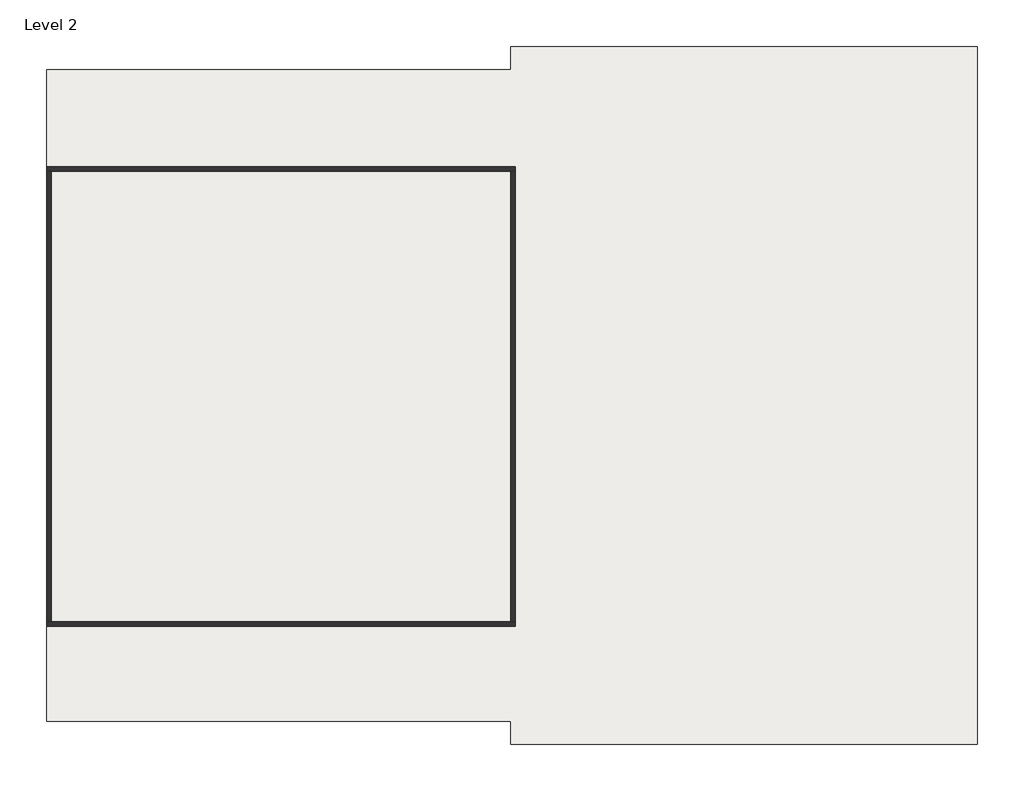
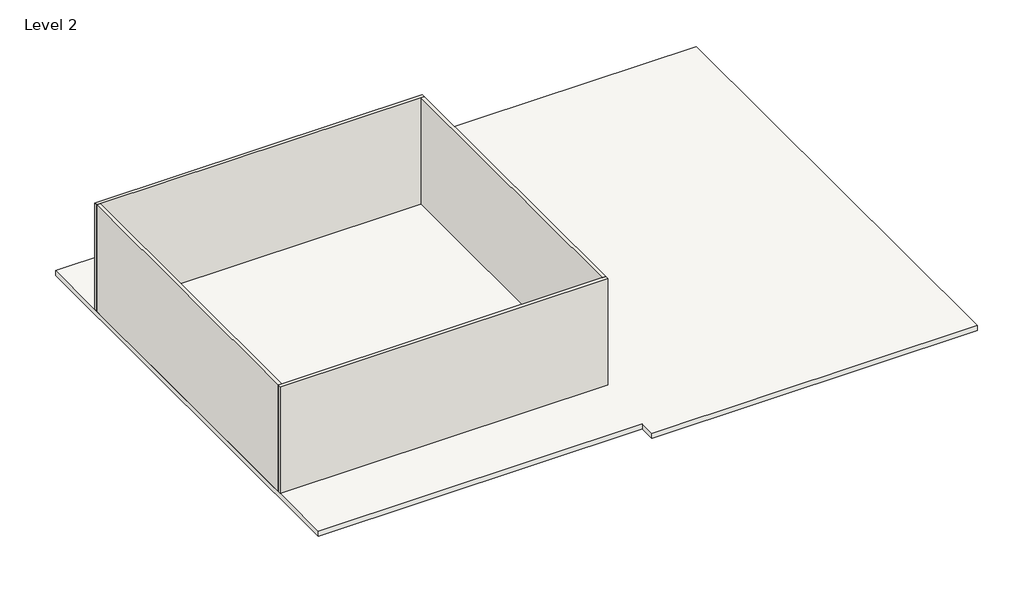
# One storey: 4 walls, 1 slab.
"""IFC4 building model written with IfcOpenShell, lengths in millimetres."""

from ifc_helpers import new_model, si_unit, frame, origin, place, context, project, spatial, polyline, outline, extrude, faceted_brep, element, save

model = new_model("IFC4")

# Units and contexts
model_context = context("Model", 3, world=origin())
ifc_project = project(units=[si_unit("LENGTHUNIT", "METRE", prefix="MILLI")], contexts=[model_context])

# Site, building, storey
site = spatial("IfcSite", under=ifc_project)
building = spatial("IfcBuilding", under=site)
storey = spatial("IfcBuildingStorey", under=building, Name="Level 2", Elevation=7000.0)

# Slab
placement = place(None, origin())
element("IfcSlab", 1, ObjectType="Beam and Block 225mm Susp Ground", at=placement, inside=storey, context=model_context, shape_type="SweptSolid", body=[
    extrude(outline(polyline([(15961.6453008, 15932.1645221), (15961.6453008, 16932.1645221), (36161.6453008, 16932.1645221), (36161.6453008, -13267.8354779), (15961.6453008, -13267.8354779), (15961.6453008, -12267.8354779), (-4138.8546992, -12267.8354779), (-4138.8546992, 15932.1645221), (15961.6453008, 15932.1645221)])), frame((0.0, 0.0, 6680.0), z_axis=(0.0, 0.0, 1.0), x_axis=(1.0, 0.0, 0.0)), (0.0, 0.0, 1.0), 320.0),
])

# Walls
element("IfcWall", 2, ObjectType="curtain wall - 200mm", at=placement, inside=storey, context=model_context, shape_type="Brep", body=[
    faceted_brep([(-4138.8546992, -8167.8354779, 7000.0), (16161.6453008, -8167.8354779, 7000.0), (16161.6453008, -8167.8354779, 14000.0), (-4138.8546992, -8167.8354779, 14000.0), (-4138.8546992, -7967.8354779, 7000.0), (-4138.8546992, -7967.8354779, 14000.0), (-3938.8546992, -7967.8354779, 14000.0), (15961.6453008, -7967.8354779, 14000.0), (16161.6453008, -7967.8354779, 14000.0), (16161.6453008, -7967.8354779, 7000.0), (15961.6453008, -7967.8354779, 7000.0), (-3938.8546992, -7967.8354779, 7000.0)], [[[0, 1, 2, 3]], [[4, 5, 6, 7, 8, 9, 10, 11]], [[1, 0, 4, 11, 10, 9]], [[3, 2, 8, 7, 6, 5]], [[2, 1, 9, 8]], [[0, 3, 5, 4]]]),
])
element("IfcWall", 3, ObjectType="curtain wall - 200mm", at=placement, inside=storey, context=model_context, shape_type="Brep", body=[
    faceted_brep([(-4138.8546992, 11532.1645221, 7000.0), (-3938.8546992, 11532.1645221, 7000.0), (15961.6453008, 11532.1645221, 7000.0), (16161.6453008, 11532.1645221, 7000.0), (16161.6453008, 11532.1645221, 14000.0), (15961.6453008, 11532.1645221, 14000.0), (-3938.8546992, 11532.1645221, 14000.0), (-4138.8546992, 11532.1645221, 14000.0), (-4138.8546992, 11732.1645221, 7000.0), (-4138.8546992, 11732.1645221, 14000.0), (16161.6453008, 11732.1645221, 14000.0), (16161.6453008, 11732.1645221, 7000.0)], [[[0, 1, 2, 3, 4, 5, 6, 7]], [[8, 9, 10, 11]], [[3, 2, 1, 0, 8, 11]], [[7, 6, 5, 4, 10, 9]], [[4, 3, 11, 10]], [[0, 7, 9, 8]]]),
])
element("IfcWall", 4, ObjectType="curtain wall - 200mm", at=placement, inside=storey, context=model_context, shape_type="SweptSolid", body=[
    extrude(outline(polyline([(15961.6453008, -7967.8354779), (15961.6453008, 11532.1645221), (16161.6453008, 11532.1645221), (16161.6453008, -7967.8354779), (15961.6453008, -7967.8354779)])), frame((0.0, 0.0, 7000.0), z_axis=(0.0, 0.0, 1.0), x_axis=(1.0, 0.0, 0.0)), (0.0, 0.0, 1.0), 7000.0),
])
element("IfcWall", 5, ObjectType="curtain wall - 200mm", at=placement, inside=storey, context=model_context, shape_type="SweptSolid", body=[
    extrude(outline(polyline([(-4138.8546992, -7967.8354779), (-4138.8546992, 11532.1645221), (-3938.8546992, 11532.1645221), (-3938.8546992, -7967.8354779), (-4138.8546992, -7967.8354779)])), frame((0.0, 0.0, 7000.0), z_axis=(0.0, 0.0, 1.0), x_axis=(1.0, 0.0, 0.0)), (0.0, 0.0, 1.0), 7000.0),
])

save(model, "model.ifc")

# Revit data of these elements
# Type "Beam and Block 225mm Susp Ground"
#   Keynote = "E60/130"
#   Function = 0
#   Layers, outside or top first: 65 mm "Concrete, Sand/Cement Screed" (function 4); 0 mm "Vapor Retarder" (function 100); 80 mm "Rigid insulation" (function 3); 0 mm "Damp-proofing" (function 100); 100 mm "Concrete Masonry, Floor Block" (function 1); 75 mm "Concrete, Precast" (function 1)
# Type "curtain wall - 200mm"
#   Layers, outside or top first: 200 mm "Glass, Clear Glazing" (function 1)
# Element 1 (IfcSlab, "Beam and Block 225mm Susp Ground")
#   Height Offset From Level = 0 mm
#   Phase Created = New Construction
#   Materials on its faces: "Concrete, Precast", "Concrete, Sand/Cement Screed"
# Elements 2, 3, 4, 5 (IfcWall, "curtain wall - 200mm")
#   Top Offset = 0 mm
#   Base Offset = 0 mm
#   wall height = 7000 mm
#   Phase Created = New Construction
#   Base Constraint = Level 2
#   Top Constraint = Roof Level
#   Materials on its faces: "Glass, Clear Glazing"
# Materials
#   "Concrete, Sand/Cement Screed": class "Concrete", colour RGB 127 127 127, transparency 0, Description = "Concrete slab topping", Cost = 0
#   "Vapor Retarder": class "Generic", colour RGB 120 120 120, transparency 0, Description = "Polyethylene film membrane", Cost = 0
#   "Rigid insulation": class "Generic", colour RGB 127 127 127, transparency 0, Description = "Rigid foam insulation board", Cost = 0
#   "Damp-proofing": class "Generic", colour RGB 127 127 127, transparency 0, Description = "Damp-proofing", Cost = 0
#   "Concrete Masonry, Floor Block": class "Concrete", colour RGB 181 181 181, transparency 0, Description = "physical material", Cost = 0
#   "Concrete, Precast": class "Concrete", colour RGB 192 192 192, transparency 0, Description = "Precast concrete", Cost = 0
#   "Glass, Clear Glazing": class "Glass", colour RGB 0 128 192, transparency 0.75, Description = "Clear glazing", Cost = 0
# Room at (5992.168, 1548.848) mm, phase "New Construction", upper level "Level 2", upper offset 7515 mm, lower offset 0 mm
#   Number = "5"
#   Name = "Room"
